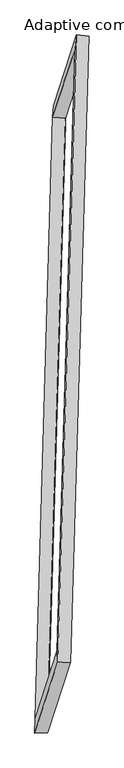
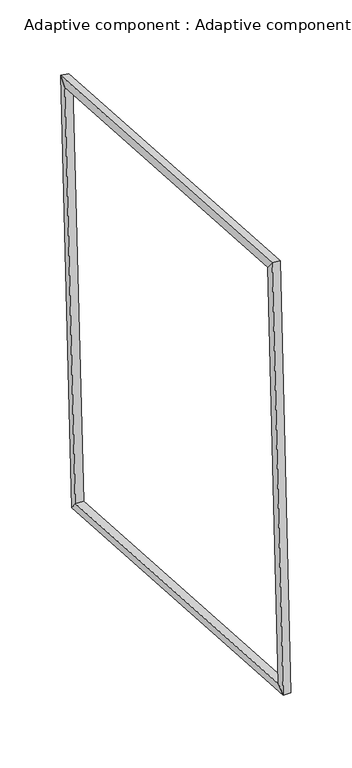
"""IFC4 building model written with IfcOpenShell, lengths in millimetres: proxy geometry, Adaptive component : Adaptive component."""

from ifc_helpers import new_model, si_unit, origin, place, context, project, spatial, faceted_brep, source, transform, mapped, element, save


def adaptive_component_adaptive_component_6dc545f0(model_context):
    return source(origin(), model_context, "Body", "Brep", [
        faceted_brep([(77.3817429, 1268.192936, 2867.0998135), (142.0173148, 1262.3512134, 2862.1411844), (51.9696717, -1762.9456122, 3174.2220617), (-12.8663677, -1763.8389201, 3179.8754571), (84.832258, 1339.216481, 2924.8810822), (-9.2579515, -1821.8969285, 3250.9724058), (149.4678299, 1333.3747584, 2919.9224531), (55.5780879, -1821.0036206, 3245.3190104), (-59.3349343, -2104.9567858, -173.3333682), (-124.3949084, -2106.538189, -174.4149488), (-125.0783569, -2177.7840227, -232.3985085), (-60.0183828, -2176.2026196, -231.3169279), (30.7127089, 920.3400397, -485.4142455), (-34.1467977, 925.4936671, -487.1905924), (-30.9881474, 983.3293867, -558.4898321), (33.8713592, 978.1757594, -556.7134852)], [[[0, 1, 2, 3]], [[4, 0, 3, 5]], [[6, 4, 5, 7]], [[1, 6, 7, 2]], [[3, 2, 8, 9]], [[5, 3, 9, 10]], [[7, 5, 10, 11]], [[2, 7, 11, 8]], [[9, 8, 12, 13]], [[10, 9, 13, 14]], [[11, 10, 14, 15]], [[8, 11, 15, 12]], [[13, 12, 1, 0]], [[14, 13, 0, 4]], [[15, 14, 4, 6]], [[12, 15, 6, 1]]]),
    ])


if __name__ == "__main__":
    model = new_model("IFC4")
    model_context = context("Model", 3, world=origin())
    ifc_project = project(units=[si_unit("LENGTHUNIT", "METRE", prefix="MILLI")], contexts=[model_context])
    site = spatial("IfcSite", under=ifc_project)
    building = spatial("IfcBuilding", under=site)
    placement = place(None, origin())
    adaptive_component_adaptive_component_shape = adaptive_component_adaptive_component_6dc545f0(model_context)
    element("IfcBuildingElementProxy", 1, Name="Adaptive component : Adaptive component", ObjectType="Adaptive component : Adaptive component", at=placement, inside=building, context=model_context, shape_type="MappedRepresentation", body=[
        mapped(adaptive_component_adaptive_component_shape, transform((0.0, 0.0, 0.0), x_axis=(1.0, 0.0, 0.0), y_axis=(0.0, 1.0, 0.0), z_axis=(0.0, 0.0, 1.0))),
    ])
    save(model, "model.ifc")

# Revit data of these elements
# Type "Adaptive component : Adaptive component"
#   r [instance default] = 2063.125 mm
#   2r [instance default] = 4126.251 mm
#   Number [instance default] = 5
#   Default Elevation = 0
# Element 1 (IfcBuildingElementProxy, "Adaptive component : Adaptive component")
#   r = 2363.054 mm
#   2r = 4726.108 mm
#   Number = 16
